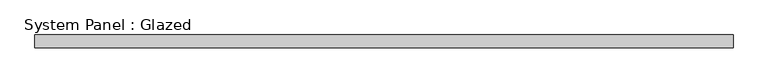
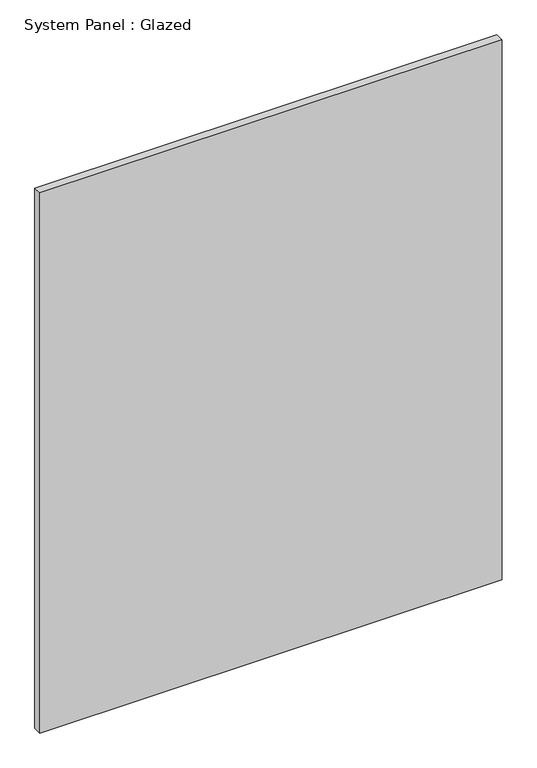
"""IFC4 building model written with IfcOpenShell, lengths in millimetres: plate geometry, System Panel : Glazed."""

from ifc_helpers import new_model, si_unit, origin, origin_with_axes, place, context, project, spatial, polyline, outline, extrude, source, transform, mapped, element, save


def system_panel_glazed_38450536(model_context):
    return source(origin(), model_context, "Body", "SweptSolid", [
        extrude(outline(polyline([(682.4999998, 24.5), (-682.4999998, 24.5), (-682.4999998, 49.5), (682.4999998, 49.5), (682.4999998, 24.5)])), origin_with_axes(), (0.0, 0.0, 1.0), 1686.2355347),
    ])


if __name__ == "__main__":
    model = new_model("IFC4")
    model_context = context("Model", 3, world=origin())
    ifc_project = project(units=[si_unit("LENGTHUNIT", "METRE", prefix="MILLI")], contexts=[model_context])
    site = spatial("IfcSite", under=ifc_project)
    building = spatial("IfcBuilding", under=site)
    placement = place(None, origin())
    system_panel_glazed_shape = system_panel_glazed_38450536(model_context)
    element("IfcPlate", 1, ObjectType="System Panel : Glazed", at=placement, inside=building, context=model_context, shape_type="MappedRepresentation", body=[
        mapped(system_panel_glazed_shape, transform((0.0, 0.0, 0.0), x_axis=(1.0, 0.0, 0.0), y_axis=(0.0, 1.0, 0.0), z_axis=(0.0, 0.0, 1.0))),
    ])
    save(model, "model.ifc")

# Revit data of these elements
# Element 1 (IfcPlate, "System Panel : Glazed")
#   Materials on its faces: "Glass"
# Materials
#   "Glass": class "Glass", colour RGB 218 227 224, transparency 0.85, Description = "Soda Lime Glass", Cost = 0
